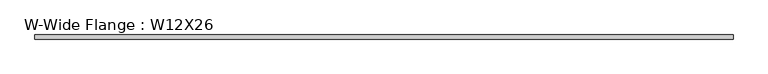
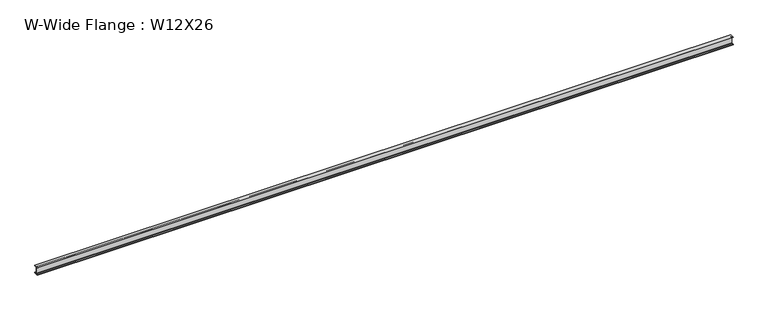
"""IFC4 building model written with IfcOpenShell, lengths in millimetres: beam geometry, W-Wide Flange : W12X26."""

from ifc_helpers import new_model, si_unit, point, frame, frame_2d, origin, place, context, project, spatial, polyline, circle_curve, trimmed, segment, composite_curve, outline, extrude, source, transform, mapped, element, save


def w_wide_flange_w12x26_79029f24(model_context):
    return source(origin(), model_context, "Body", "SweptSolid", [
        extrude(outline(composite_curve([segment(polyline([(82.4011719, -145.5539063), (82.4011719, -155.178125), (-82.4011719, -155.178125), (-82.4011719, -145.5539063), (-20.2902344, -145.5539063)]), True, "CONTINUOUS"), segment(trimmed(circle_curve(frame_2d((-20.2902344, -128.190625)), 17.3632812), [point((-20.2902344, -145.5539063))], [point((-2.9269531, -128.190625))], True, "CARTESIAN"), True, "CONTINUOUS"), segment(polyline([(-2.9269531, -128.190625), (-2.9269531, 128.190625)]), True, "CONTINUOUS"), segment(trimmed(circle_curve(frame_2d((-20.2902344, 128.190625)), 17.3632812), [point((-2.9269531, 128.190625))], [point((-20.2902344, 145.5539062))], True, "CARTESIAN"), True, "CONTINUOUS"), segment(polyline([(-20.2902344, 145.5539062), (-82.4011719, 145.5539062), (-82.4011719, 155.178125), (82.4011719, 155.178125), (82.4011719, 145.5539062), (20.2902344, 145.5539062)]), True, "CONTINUOUS"), segment(trimmed(circle_curve(frame_2d((20.2902344, 128.190625)), 17.3632812), [point((20.2902344, 145.5539062))], [point((2.9269531, 128.190625))], True, "CARTESIAN"), True, "CONTINUOUS"), segment(polyline([(2.9269531, 128.190625), (2.9269531, -128.190625)]), True, "CONTINUOUS"), segment(trimmed(circle_curve(frame_2d((20.2902344, -128.190625)), 17.3632812), [point((2.9269531, -128.190625))], [point((20.2902344, -145.5539063))], True, "CARTESIAN"), True, "CONTINUOUS"), segment(polyline([(20.2902344, -145.5539063), (82.4011719, -145.5539063)]), True, "CONTINUOUS")], self_intersect=False)), frame((-13944.6, 0.0, 0.0), z_axis=(1.0, 0.0, 0.0), x_axis=(0.0, 1.0, 0.0)), (0.0, 0.0, 1.0), 27889.2),
    ])


if __name__ == "__main__":
    model = new_model("IFC4")
    model_context = context("Model", 3, world=origin())
    ifc_project = project(units=[si_unit("LENGTHUNIT", "METRE", prefix="MILLI")], contexts=[model_context])
    site = spatial("IfcSite", under=ifc_project)
    building = spatial("IfcBuilding", under=site)
    placement = place(None, origin())
    w_wide_flange_w12x26_shape = w_wide_flange_w12x26_79029f24(model_context)
    element("IfcBeam", 1, ObjectType="W-Wide Flange : W12X26", at=placement, inside=building, context=model_context, shape_type="MappedRepresentation", body=[
        mapped(w_wide_flange_w12x26_shape, transform((0.0, 0.0, 0.0), x_axis=(1.0, 0.0, 0.0), y_axis=(0.0, 1.0, 0.0), z_axis=(0.0, 0.0, 1.0))),
    ])
    save(model, "model.ifc")

# Revit data of these elements
# Type "W-Wide Flange : W12X26"
#   Assembly Code = "B10"
#   W = 26
#   Length [instance default] = 5' - 0"
#   bf = 0' - 6 125/256"
#   d = 1' - 0 7/32"
#   k = 0' - 1 1/16"
#   k2 = 0' - 0 175/256"
#   tf = 0' - 0 97/256"
#   tw = 0' - 0 59/256"
#   A = 0.053125 SF
#   Structural Material [instance default] = none
